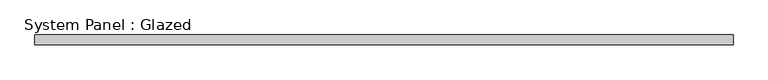
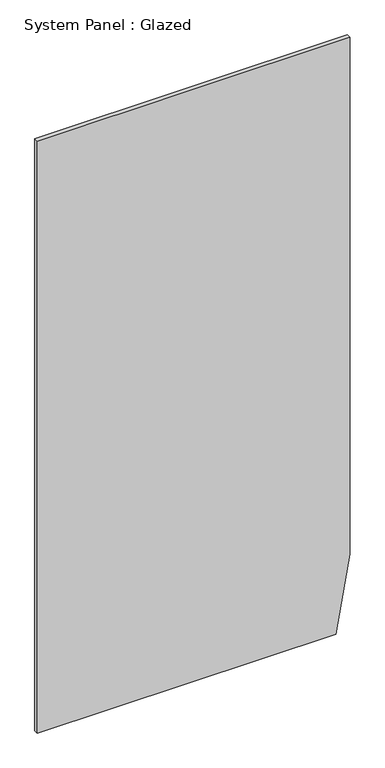
"""IFC4 building model written with IfcOpenShell, lengths in millimetres: plate geometry, System Panel : Glazed."""

import ifcopenshell
import ifcopenshell.guid

model = None  # the IFC model being written
_history = None  # IfcOwnerHistory: only IFC2X3 demands one
_inside = {}  # id of a spatial element -> (the spatial element, [elements in it])
_under = {}  # id of a project, library or spatial element -> (it, [spatial elements below it])
_declared = {}  # id of a project -> (the project, [libraries it declares])
_typed = {}  # id of a type object -> (the type object, [elements of that type])
_made_of = {}  # id of a material, layer set ... -> (it, [elements and type objects made of it])


def new_model(schema):
    """Start an empty IFC model of exactly this schema.

    Asked for "IFC4X3", IfcOpenShell would pick the latest addendum, in which some entities
    have other attributes; the version numbers below select the first issue.
    IFC2X3 requires an IfcOwnerHistory on every rooted entity: one is made here for all.
    """
    global model, _history
    if schema == "IFC4X3":
        model = ifcopenshell.file(schema_version=(4, 3, 0, 0))
    else:
        model = ifcopenshell.file(schema=schema)
    _inside.clear()
    _under.clear()
    _declared.clear()
    _typed.clear()
    _made_of.clear()
    _history = None
    if model.schema == "IFC2X3":
        org = make("IfcOrganization", Name="unknown")
        user = make(
            "IfcPersonAndOrganization",
            ThePerson=make("IfcPerson", FamilyName="unknown"),
            TheOrganization=org,
        )
        app = make(
            "IfcApplication",
            ApplicationDeveloper=org,
            Version="unknown",
            ApplicationFullName="unknown",
            ApplicationIdentifier="unknown",
        )
        _history = make(
            "IfcOwnerHistory",
            OwningUser=user,
            OwningApplication=app,
            ChangeAction="ADDED",
            CreationDate=0,
        )
    return model


def make(cls, **values):
    """One entity of the class cls with the attributes given. An attribute that is None is left unset."""
    return model.create_entity(
        cls, **{name: value for name, value in values.items() if value is not None}
    )


def rooted(cls, **values):
    """An entity with a GlobalId (a new one), such as an element, a storey or a relation."""
    return make(cls, GlobalId=ifcopenshell.guid.new(), OwnerHistory=_history, **values)


def si_unit(unit_type, name, prefix=None):
    """IfcSIUnit, for example si_unit("LENGTHUNIT", "METRE", prefix="MILLI")."""
    return make("IfcSIUnit", UnitType=unit_type, Prefix=prefix, Name=name)


def assignment(units):
    """IfcUnitAssignment: the units of a project."""
    return None if units is None else make("IfcUnitAssignment", Units=units)


def point(xyz):
    """IfcCartesianPoint."""
    return None if xyz is None else make("IfcCartesianPoint", Coordinates=xyz)


def direction(xyz):
    """IfcDirection."""
    return None if xyz is None else make("IfcDirection", DirectionRatios=xyz)


def frame(location, z_axis=None, x_axis=None):
    """IfcAxis2Placement3D, a coordinate frame: its origin and axes. An axis left out is left unset."""
    return make(
        "IfcAxis2Placement3D",
        Location=point(location),
        Axis=direction(z_axis),
        RefDirection=direction(x_axis),
    )


def origin():
    """The frame at (0, 0, 0) with its axes left unset."""
    return frame((0.0, 0.0, 0.0))


def place(relative_to, where):
    """IfcLocalPlacement: puts the frame where relative to a parent placement (None: the world)."""
    return make(
        "IfcLocalPlacement", PlacementRelTo=relative_to, RelativePlacement=where
    )


def context(
    kind, dimensions, precision=None, world=None, true_north=None, identifier=None
):
    """IfcGeometricRepresentationContext, for example the 3D "Model" context."""
    return make(
        "IfcGeometricRepresentationContext",
        ContextIdentifier=identifier,
        ContextType=kind,
        CoordinateSpaceDimension=dimensions,
        Precision=precision,
        WorldCoordinateSystem=world,
        TrueNorth=true_north,
    )


def project(units=None, contexts=None):
    """IfcProject with its units and contexts."""
    return rooted(
        "IfcProject",
        Name="project",
        RepresentationContexts=contexts,
        UnitsInContext=assignment(units),
    )


def spatial(cls, under=None, at=None, **own):
    """A site, building, storey or space (cls), placed at a placement, below another one or the project."""
    s = rooted(cls, ObjectPlacement=at, **own)
    if under is not None:
        _under.setdefault(under.id(), (under, []))[1].append(s)
    return s


def polyline(points):
    """IfcPolyline through the points."""
    return make("IfcPolyline", Points=[point(p) for p in points])


def outline(outer, holes=None, kind="AREA"):
    """IfcArbitraryClosedProfileDef: a profile drawn as a closed curve; with holes, ...WithVoids."""
    if holes is None:
        return make("IfcArbitraryClosedProfileDef", ProfileType=kind, OuterCurve=outer)
    return make(
        "IfcArbitraryProfileDefWithVoids",
        ProfileType=kind,
        OuterCurve=outer,
        InnerCurves=holes,
    )


def extrude(swept, where, along, depth):
    """IfcExtrudedAreaSolid: the profile swept, set in the frame where, extruded along a direction by depth."""
    return make(
        "IfcExtrudedAreaSolid",
        SweptArea=swept,
        Position=where,
        ExtrudedDirection=direction(along),
        Depth=depth,
    )


def shape(context_of_items, identifier, shape_type, items):
    """IfcShapeRepresentation: the items that make up one representation, for example the "Body"."""
    return make(
        "IfcShapeRepresentation",
        ContextOfItems=context_of_items,
        RepresentationIdentifier=identifier,
        RepresentationType=shape_type,
        Items=items,
    )


def source(mapping_origin, context_of_items, identifier, shape_type, items):
    """IfcRepresentationMap: a shape defined once, which mapped items show again and again."""
    return make(
        "IfcRepresentationMap",
        MappingOrigin=mapping_origin,
        MappedRepresentation=shape(context_of_items, identifier, shape_type, items),
    )


def transform(
    local_origin,
    x_axis=None,
    y_axis=None,
    z_axis=None,
    scale=None,
    scale2=None,
    scale3=None,
    uniform=True,
):
    """IfcCartesianTransformationOperator3D, or its non-uniform kind. x_axis, y_axis, z_axis: its Axis1, 2, 3."""
    if uniform:
        return make(
            "IfcCartesianTransformationOperator3D",
            Axis1=direction(x_axis),
            Axis2=direction(y_axis),
            LocalOrigin=point(local_origin),
            Scale=scale,
            Axis3=direction(z_axis),
        )
    return make(
        "IfcCartesianTransformationOperator3DnonUniform",
        Axis1=direction(x_axis),
        Axis2=direction(y_axis),
        LocalOrigin=point(local_origin),
        Scale=scale,
        Axis3=direction(z_axis),
        Scale2=scale2,
        Scale3=scale3,
    )


def mapped(mapping_source, mapping_target):
    """IfcMappedItem: shows the shape of a source again, moved by a transform."""
    return make(
        "IfcMappedItem", MappingSource=mapping_source, MappingTarget=mapping_target
    )


def made_of(thing, what):
    """Note that an element or type object is made of a material, layer set ...; save() writes the relation."""
    if what is not None:
        _made_of.setdefault(what.id(), (what, []))[1].append(thing)
    return thing


def element(
    cls,
    number,
    at=None,
    inside=None,
    cuts=None,
    type_object=None,
    material=None,
    context=None,
    identifier="Body",
    shape_type=None,
    held_by="IfcProductDefinitionShape",
    body=None,
    shapes=None,
    **own,
):
    """One element of the class cls, such as IfcWall. Its Tag is "e" and its number.

    at: its placement. inside: the storey or other place that contains it. cuts: it is an
    opening in that element (IfcRelVoidsElement). A single representation is given by context,
    identifier, shape_type and body (its items); several are given by shapes. held_by: the class
    of the entity that holds the representations. save() writes the other relations.
    """
    e = rooted(cls, Tag="e%d" % number, ObjectPlacement=at, **own)
    if body is not None:
        shapes = [shape(context, identifier, shape_type, body)]
    if shapes is not None:
        e.Representation = make(held_by, Representations=shapes)
    if inside is not None:
        _inside.setdefault(inside.id(), (inside, []))[1].append(e)
    if cuts is not None:
        rooted(
            "IfcRelVoidsElement", RelatingBuildingElement=cuts, RelatedOpeningElement=e
        )
    if type_object is not None:
        _typed.setdefault(type_object.id(), (type_object, []))[1].append(e)
    return made_of(e, material)


def aggregate(whole, parts):
    """IfcRelAggregates: a whole, such as a stair, and the parts it consists of."""
    return rooted("IfcRelAggregates", RelatingObject=whole, RelatedObjects=parts)


def save(model, path):
    """Write the relations noted so far, then the file.

    IfcRelAggregates (storeys below a building ...), IfcRelContainedInSpatialStructure (elements
    in a storey), IfcRelDefinesByType, IfcRelAssociatesMaterial and IfcRelDeclares: one each for
    every whole, place, type object, material and project.
    """
    for whole, parts in _under.values():
        aggregate(whole, parts)
    for where, things in _inside.values():
        rooted(
            "IfcRelContainedInSpatialStructure",
            RelatedElements=things,
            RelatingStructure=where,
        )
    for kind, things in _typed.values():
        rooted("IfcRelDefinesByType", RelatedObjects=things, RelatingType=kind)
    for what, things in _made_of.values():
        rooted("IfcRelAssociatesMaterial", RelatedObjects=things, RelatingMaterial=what)
    for by, libraries in _declared.values():
        rooted("IfcRelDeclares", RelatingContext=by, RelatedDefinitions=libraries)
    model.write(path)


def system_panel_glazed_959d3605(model_context):
    return source(origin(), model_context, "Body", "SweptSolid", [
        extrude(outline(polyline([(0.0, -914.4), (0.0, 832.7834794), (464.6383785, 914.4), (3657.6, 914.4), (3657.6, -914.4), (0.0, -914.4)])), frame((0.0, -44.45, 0.0), z_axis=(0.0, 1.0, 0.0), x_axis=(0.0, 0.0, 1.0)), (0.0, 0.0, 1.0), 25.4),
    ])


if __name__ == "__main__":
    model = new_model("IFC4")
    model_context = context("Model", 3, world=origin())
    ifc_project = project(units=[si_unit("LENGTHUNIT", "METRE", prefix="MILLI")], contexts=[model_context])
    site = spatial("IfcSite", under=ifc_project)
    building = spatial("IfcBuilding", under=site)
    placement = place(None, origin())
    system_panel_glazed_shape = system_panel_glazed_959d3605(model_context)
    element("IfcPlate", 1, ObjectType="System Panel : Glazed", at=placement, inside=building, context=model_context, shape_type="MappedRepresentation", body=[
        mapped(system_panel_glazed_shape, transform((0.0, 0.0, 0.0), x_axis=(1.0, 0.0, 0.0), y_axis=(0.0, 1.0, 0.0), z_axis=(0.0, 0.0, 1.0))),
    ])
    save(model, "model.ifc")

# Revit data of these elements
# Type "System Panel : Glazed"
#   Construction Type Id = "GSP4R"
#   Analytic Construction = "1/8 in Pilkington single glazing"
#   Visual Light Transmittance = 0.9
#   Solar Heat Gain Coefficient = 0.86
#   Heat Transfer Coefficient (U) = 1.18115 BTU/(h·ft²·°F)
#   Define Thermal Properties by = 1
# Element 1 (IfcPlate, "System Panel : Glazed")
#   Materials on its faces: "Glass"
# Materials
#   "Glass": class "Glass", colour RGB 0 128 192, transparency 0.75, Description = "Soda Lime Glass", Cost = 0
